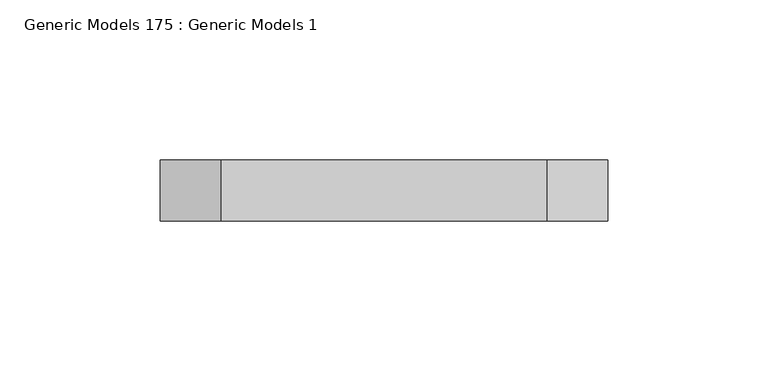
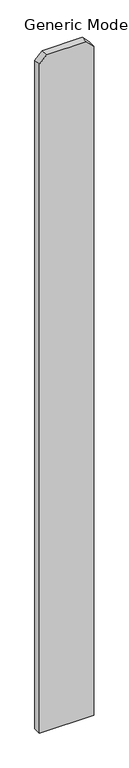
"""IFC4 building model written with IfcOpenShell, lengths in millimetres: proxy geometry, Generic Models 175 : Generic Models 1."""

import ifcopenshell
import ifcopenshell.guid

model = None  # the IFC model being written
_history = None  # IfcOwnerHistory: only IFC2X3 demands one
_inside = {}  # id of a spatial element -> (the spatial element, [elements in it])
_under = {}  # id of a project, library or spatial element -> (it, [spatial elements below it])
_declared = {}  # id of a project -> (the project, [libraries it declares])
_typed = {}  # id of a type object -> (the type object, [elements of that type])
_made_of = {}  # id of a material, layer set ... -> (it, [elements and type objects made of it])


def new_model(schema):
    """Start an empty IFC model of exactly this schema.

    Asked for "IFC4X3", IfcOpenShell would pick the latest addendum, in which some entities
    have other attributes; the version numbers below select the first issue.
    IFC2X3 requires an IfcOwnerHistory on every rooted entity: one is made here for all.
    """
    global model, _history
    if schema == "IFC4X3":
        model = ifcopenshell.file(schema_version=(4, 3, 0, 0))
    else:
        model = ifcopenshell.file(schema=schema)
    _inside.clear()
    _under.clear()
    _declared.clear()
    _typed.clear()
    _made_of.clear()
    _history = None
    if model.schema == "IFC2X3":
        org = make("IfcOrganization", Name="unknown")
        user = make(
            "IfcPersonAndOrganization",
            ThePerson=make("IfcPerson", FamilyName="unknown"),
            TheOrganization=org,
        )
        app = make(
            "IfcApplication",
            ApplicationDeveloper=org,
            Version="unknown",
            ApplicationFullName="unknown",
            ApplicationIdentifier="unknown",
        )
        _history = make(
            "IfcOwnerHistory",
            OwningUser=user,
            OwningApplication=app,
            ChangeAction="ADDED",
            CreationDate=0,
        )
    return model


def make(cls, **values):
    """One entity of the class cls with the attributes given. An attribute that is None is left unset."""
    return model.create_entity(
        cls, **{name: value for name, value in values.items() if value is not None}
    )


def rooted(cls, **values):
    """An entity with a GlobalId (a new one), such as an element, a storey or a relation."""
    return make(cls, GlobalId=ifcopenshell.guid.new(), OwnerHistory=_history, **values)


def si_unit(unit_type, name, prefix=None):
    """IfcSIUnit, for example si_unit("LENGTHUNIT", "METRE", prefix="MILLI")."""
    return make("IfcSIUnit", UnitType=unit_type, Prefix=prefix, Name=name)


def assignment(units):
    """IfcUnitAssignment: the units of a project."""
    return None if units is None else make("IfcUnitAssignment", Units=units)


def point(xyz):
    """IfcCartesianPoint."""
    return None if xyz is None else make("IfcCartesianPoint", Coordinates=xyz)


def direction(xyz):
    """IfcDirection."""
    return None if xyz is None else make("IfcDirection", DirectionRatios=xyz)


def frame(location, z_axis=None, x_axis=None):
    """IfcAxis2Placement3D, a coordinate frame: its origin and axes. An axis left out is left unset."""
    return make(
        "IfcAxis2Placement3D",
        Location=point(location),
        Axis=direction(z_axis),
        RefDirection=direction(x_axis),
    )


def origin():
    """The frame at (0, 0, 0) with its axes left unset."""
    return frame((0.0, 0.0, 0.0))


def place(relative_to, where):
    """IfcLocalPlacement: puts the frame where relative to a parent placement (None: the world)."""
    return make(
        "IfcLocalPlacement", PlacementRelTo=relative_to, RelativePlacement=where
    )


def context(
    kind, dimensions, precision=None, world=None, true_north=None, identifier=None
):
    """IfcGeometricRepresentationContext, for example the 3D "Model" context."""
    return make(
        "IfcGeometricRepresentationContext",
        ContextIdentifier=identifier,
        ContextType=kind,
        CoordinateSpaceDimension=dimensions,
        Precision=precision,
        WorldCoordinateSystem=world,
        TrueNorth=true_north,
    )


def project(units=None, contexts=None):
    """IfcProject with its units and contexts."""
    return rooted(
        "IfcProject",
        Name="project",
        RepresentationContexts=contexts,
        UnitsInContext=assignment(units),
    )


def spatial(cls, under=None, at=None, **own):
    """A site, building, storey or space (cls), placed at a placement, below another one or the project."""
    s = rooted(cls, ObjectPlacement=at, **own)
    if under is not None:
        _under.setdefault(under.id(), (under, []))[1].append(s)
    return s


def polyline(points):
    """IfcPolyline through the points."""
    return make("IfcPolyline", Points=[point(p) for p in points])


def outline(outer, holes=None, kind="AREA"):
    """IfcArbitraryClosedProfileDef: a profile drawn as a closed curve; with holes, ...WithVoids."""
    if holes is None:
        return make("IfcArbitraryClosedProfileDef", ProfileType=kind, OuterCurve=outer)
    return make(
        "IfcArbitraryProfileDefWithVoids",
        ProfileType=kind,
        OuterCurve=outer,
        InnerCurves=holes,
    )


def extrude(swept, where, along, depth):
    """IfcExtrudedAreaSolid: the profile swept, set in the frame where, extruded along a direction by depth."""
    return make(
        "IfcExtrudedAreaSolid",
        SweptArea=swept,
        Position=where,
        ExtrudedDirection=direction(along),
        Depth=depth,
    )


def shape(context_of_items, identifier, shape_type, items):
    """IfcShapeRepresentation: the items that make up one representation, for example the "Body"."""
    return make(
        "IfcShapeRepresentation",
        ContextOfItems=context_of_items,
        RepresentationIdentifier=identifier,
        RepresentationType=shape_type,
        Items=items,
    )


def source(mapping_origin, context_of_items, identifier, shape_type, items):
    """IfcRepresentationMap: a shape defined once, which mapped items show again and again."""
    return make(
        "IfcRepresentationMap",
        MappingOrigin=mapping_origin,
        MappedRepresentation=shape(context_of_items, identifier, shape_type, items),
    )


def transform(
    local_origin,
    x_axis=None,
    y_axis=None,
    z_axis=None,
    scale=None,
    scale2=None,
    scale3=None,
    uniform=True,
):
    """IfcCartesianTransformationOperator3D, or its non-uniform kind. x_axis, y_axis, z_axis: its Axis1, 2, 3."""
    if uniform:
        return make(
            "IfcCartesianTransformationOperator3D",
            Axis1=direction(x_axis),
            Axis2=direction(y_axis),
            LocalOrigin=point(local_origin),
            Scale=scale,
            Axis3=direction(z_axis),
        )
    return make(
        "IfcCartesianTransformationOperator3DnonUniform",
        Axis1=direction(x_axis),
        Axis2=direction(y_axis),
        LocalOrigin=point(local_origin),
        Scale=scale,
        Axis3=direction(z_axis),
        Scale2=scale2,
        Scale3=scale3,
    )


def mapped(mapping_source, mapping_target):
    """IfcMappedItem: shows the shape of a source again, moved by a transform."""
    return make(
        "IfcMappedItem", MappingSource=mapping_source, MappingTarget=mapping_target
    )


def made_of(thing, what):
    """Note that an element or type object is made of a material, layer set ...; save() writes the relation."""
    if what is not None:
        _made_of.setdefault(what.id(), (what, []))[1].append(thing)
    return thing


def element(
    cls,
    number,
    at=None,
    inside=None,
    cuts=None,
    type_object=None,
    material=None,
    context=None,
    identifier="Body",
    shape_type=None,
    held_by="IfcProductDefinitionShape",
    body=None,
    shapes=None,
    **own,
):
    """One element of the class cls, such as IfcWall. Its Tag is "e" and its number.

    at: its placement. inside: the storey or other place that contains it. cuts: it is an
    opening in that element (IfcRelVoidsElement). A single representation is given by context,
    identifier, shape_type and body (its items); several are given by shapes. held_by: the class
    of the entity that holds the representations. save() writes the other relations.
    """
    e = rooted(cls, Tag="e%d" % number, ObjectPlacement=at, **own)
    if body is not None:
        shapes = [shape(context, identifier, shape_type, body)]
    if shapes is not None:
        e.Representation = make(held_by, Representations=shapes)
    if inside is not None:
        _inside.setdefault(inside.id(), (inside, []))[1].append(e)
    if cuts is not None:
        rooted(
            "IfcRelVoidsElement", RelatingBuildingElement=cuts, RelatedOpeningElement=e
        )
    if type_object is not None:
        _typed.setdefault(type_object.id(), (type_object, []))[1].append(e)
    return made_of(e, material)


def aggregate(whole, parts):
    """IfcRelAggregates: a whole, such as a stair, and the parts it consists of."""
    return rooted("IfcRelAggregates", RelatingObject=whole, RelatedObjects=parts)


def save(model, path):
    """Write the relations noted so far, then the file.

    IfcRelAggregates (storeys below a building ...), IfcRelContainedInSpatialStructure (elements
    in a storey), IfcRelDefinesByType, IfcRelAssociatesMaterial and IfcRelDeclares: one each for
    every whole, place, type object, material and project.
    """
    for whole, parts in _under.values():
        aggregate(whole, parts)
    for where, things in _inside.values():
        rooted(
            "IfcRelContainedInSpatialStructure",
            RelatedElements=things,
            RelatingStructure=where,
        )
    for kind, things in _typed.values():
        rooted("IfcRelDefinesByType", RelatedObjects=things, RelatingType=kind)
    for what, things in _made_of.values():
        rooted("IfcRelAssociatesMaterial", RelatedObjects=things, RelatingMaterial=what)
    for by, libraries in _declared.values():
        rooted("IfcRelDeclares", RelatingContext=by, RelatedDefinitions=libraries)
    model.write(path)


def generic_models_175_generic_models_1_782693d9(model_context):
    return source(origin(), model_context, "Body", "SweptSolid", [
        extrude(outline(polyline([(76.2, 56665.8125), (1885.95, 56665.8125), (1905.0, 56646.7625), (1905.0, 56545.1625), (1885.95, 56526.1125), (76.2, 56526.1125), (76.2, 56665.8125)])), frame((0.0, 547.6875, 0.0), z_axis=(0.0, 1.0, 0.0), x_axis=(0.0, 0.0, 1.0)), (0.0, 0.0, 1.0), 19.05),
    ])


if __name__ == "__main__":
    model = new_model("IFC4")
    model_context = context("Model", 3, world=origin())
    ifc_project = project(units=[si_unit("LENGTHUNIT", "METRE", prefix="MILLI")], contexts=[model_context])
    site = spatial("IfcSite", under=ifc_project)
    building = spatial("IfcBuilding", under=site)
    placement = place(None, origin())
    generic_models_175_generic_models_1_shape = generic_models_175_generic_models_1_782693d9(model_context)
    element("IfcBuildingElementProxy", 1, Name="Generic Models 175 : Generic Models 1", ObjectType="Generic Models 175 : Generic Models 1", at=placement, inside=building, context=model_context, shape_type="MappedRepresentation", body=[
        mapped(generic_models_175_generic_models_1_shape, transform((0.0, 0.0, 0.0), x_axis=(1.0, 0.0, 0.0), y_axis=(0.0, 1.0, 0.0), z_axis=(0.0, 0.0, 1.0))),
    ])
    save(model, "model.ifc")

# Revit data of these elements
# Element 1 (IfcBuildingElementProxy, "Generic Models 175 : Generic Models 1")
#   Materials on its faces: "VERTICAL 1X6 CEDAR PLANKS W/ CLEAR WOOD SEALER"
# Materials
#   "VERTICAL 1X6 CEDAR PLANKS W/ CLEAR WOOD SEALER": class "Wood", colour RGB 234 198 147, transparency 0, Description = "Pinus Echinata", Cost = 0
